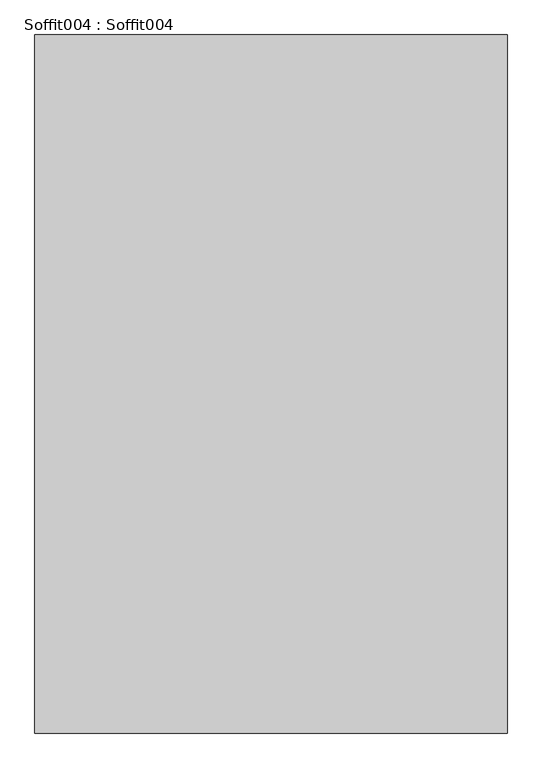
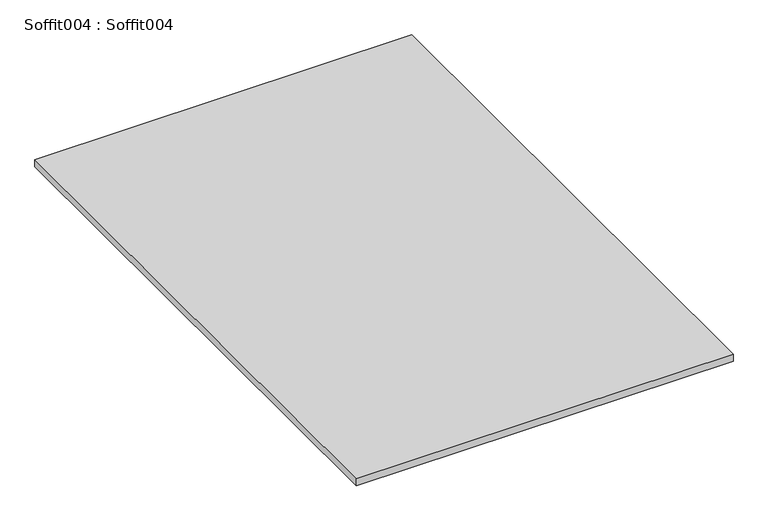
"""IFC4 building model written with IfcOpenShell, lengths in millimetres: proxy geometry, Soffit004 : Soffit004."""

from ifc_helpers import new_model, si_unit, frame, origin, place, context, project, spatial, polyline, outline, extrude, source, transform, mapped, element, save


def soffit004_soffit004_7ee9a360(model_context):
    return source(origin(), model_context, "Body", "SweptSolid", [
        extrude(outline(polyline([(-1098.3786621, -1052.8906574), (-2452.3324643, -1052.8906574), (-2452.3324643, 947.1093426), (-1098.3786621, 947.1093426), (-1098.3786621, -1052.8906574)])), frame((0.0, 0.0, 42101.9016246), z_axis=(0.0, 0.0, 1.0), x_axis=(1.0, 0.0, 0.0)), (0.0, 0.0, 1.0), 26.0465759),
    ])


if __name__ == "__main__":
    model = new_model("IFC4")
    model_context = context("Model", 3, world=origin())
    ifc_project = project(units=[si_unit("LENGTHUNIT", "METRE", prefix="MILLI")], contexts=[model_context])
    site = spatial("IfcSite", under=ifc_project)
    building = spatial("IfcBuilding", under=site)
    placement = place(None, origin())
    soffit004_soffit004_shape = soffit004_soffit004_7ee9a360(model_context)
    element("IfcBuildingElementProxy", 1, Name="Soffit004 : Soffit004", ObjectType="Soffit004 : Soffit004", at=placement, inside=building, context=model_context, shape_type="MappedRepresentation", body=[
        mapped(soffit004_soffit004_shape, transform((0.0, 0.0, 0.0), x_axis=(1.0, 0.0, 0.0), y_axis=(0.0, 1.0, 0.0), z_axis=(0.0, 0.0, 1.0))),
    ])
    save(model, "model.ifc")

# Revit data of these elements
# Type "Soffit004 : Soffit004"
#   NameOverride = "Soffit004"
# Element 1 (IfcBuildingElementProxy, "Soffit004 : Soffit004")
#   Materials on its faces: "WHITE OAK OVER BUILDING WRAP"
# Materials
#   "WHITE OAK OVER BUILDING WRAP": class "Unassigned", colour RGB 227 188 136, transparency 0, Cost = 0
